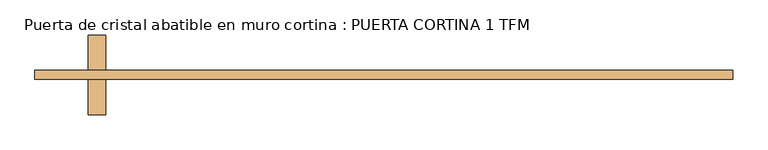
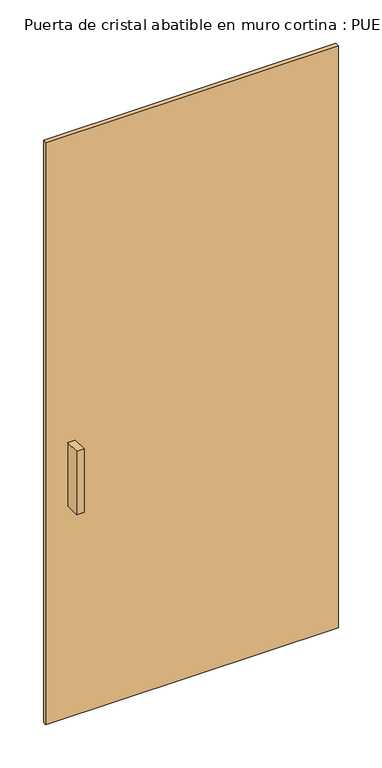
"""IFC4 building model written with IfcOpenShell, lengths in millimetres: door geometry, Puerta de cristal abatible en muro cortina : PUERTA CORTINA 1 TFM."""

from ifc_helpers import new_model, si_unit, frame, origin, origin_with_axes, place, context, project, spatial, polyline, outline, extrude, source, transform, mapped, element, save


def puerta_de_cristal_abatible_en_muro_cortina_puerta_cortina_1_b4404da8(model_context):
    return source(origin(), model_context, "Body", "SweptSolid", [
        extrude(outline(polyline([(-398.4, 12.5), (-398.4, -38.3), (-423.8, -38.3), (-423.8, 12.5), (-398.4, 12.5)])), frame((0.0, 0.0, 762.0), z_axis=(0.0, 0.0, 1.0), x_axis=(1.0, 0.0, 0.0)), (0.0, 0.0, 1.0), 228.6),
        extrude(outline(polyline([(-423.8, -101.8), (-423.8, -51.0), (-398.4, -51.0), (-398.4, -101.8), (-423.8, -101.8)])), frame((0.0, 0.0, 762.0), z_axis=(0.0, 0.0, 1.0), x_axis=(1.0, 0.0, 0.0)), (0.0, 0.0, 1.0), 228.6),
        extrude(outline(polyline([(500.0, -51.0), (-500.0, -51.0), (-500.0, -38.3), (500.0, -38.3), (500.0, -51.0)])), origin_with_axes(), (0.0, 0.0, 1.0), 2100.0),
    ])


if __name__ == "__main__":
    model = new_model("IFC4")
    model_context = context("Model", 3, world=origin())
    ifc_project = project(units=[si_unit("LENGTHUNIT", "METRE", prefix="MILLI")], contexts=[model_context])
    site = spatial("IfcSite", under=ifc_project)
    building = spatial("IfcBuilding", under=site)
    placement = place(None, origin())
    puerta_de_cristal_abatible_en_muro_cortina_puerta_cortina_1_shape = puerta_de_cristal_abatible_en_muro_cortina_puerta_cortina_1_b4404da8(model_context)
    element("IfcDoor", 1, ObjectType="Puerta de cristal abatible en muro cortina : PUERTA CORTINA 1 TFM", at=placement, inside=building, context=model_context, shape_type="MappedRepresentation", body=[
        mapped(puerta_de_cristal_abatible_en_muro_cortina_puerta_cortina_1_shape, transform((0.0, 0.0, 0.0), x_axis=(1.0, 0.0, 0.0), y_axis=(0.0, 1.0, 0.0), z_axis=(0.0, 0.0, 1.0))),
    ])
    save(model, "model.ifc")

# Revit data of these elements
# Type "Puerta de cristal abatible en muro cortina : PUERTA CORTINA 1 TFM"
#   Description = "Puerta vidrio muro cortina"
#   Type Mark = "P4"
#   Construction Type Id = "SGL"
#   Analytic Construction = "Ventanas grandes con acristalamiento simple"
#   Visual Light Transmittance = 0.9
#   Solar Heat Gain Coefficient = 0.86
#   Desfase = 0.051 m
#   Heat Transfer Coefficient (U) = 5.5617 W/(m²·K)
#   Define Thermal Properties by = 1
#   Function = 1
#   Material de cristalera = Vidrio
# Element 1 (IfcDoor, "Puerta de cristal abatible en muro cortina : PUERTA CORTINA 1 TFM")
#   Materials on its faces: "Metal - Aluminio", "Vidrio"
# Materials
#   "Vidrio": class "Vidrio", colour RGB 0 128 192, transparency 0.75, Description = "Vidrio de cal sodada", Cost = 0
#   "Metal - Aluminio": class "Metal", colour RGB 247 247 247, transparency 0
